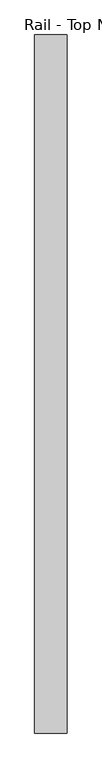
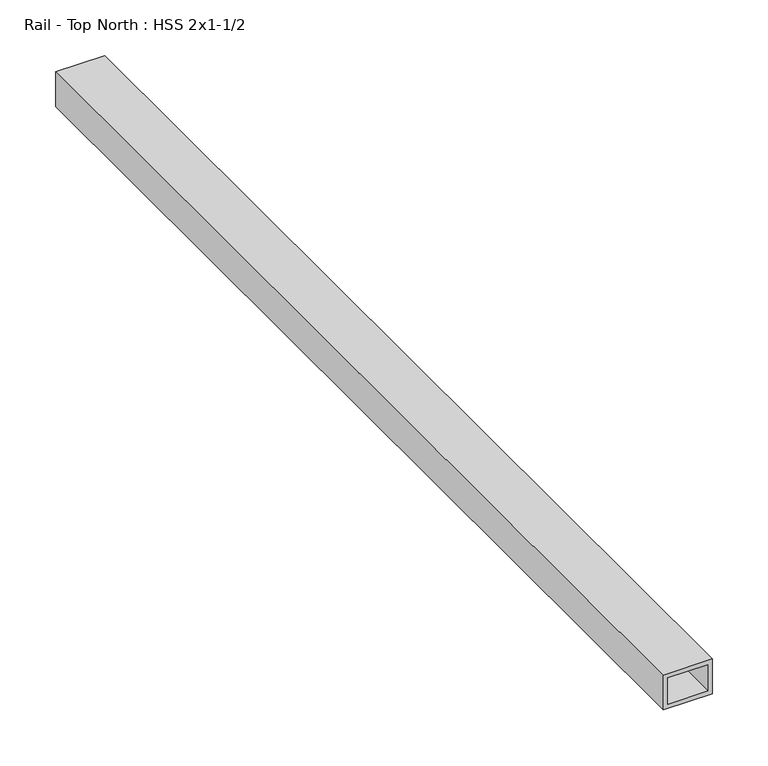
"""IFC4 building model written with IfcOpenShell, lengths in millimetres: proxy geometry, Rail - Top North : HSS 2x1-1/2."""

from ifc_helpers import new_model, si_unit, frame, origin, place, context, project, spatial, polyline, outline, extrude, source, transform, mapped, element, save


def rail_top_north_hss_2x1_1_2_493d1250(model_context):
    return source(origin(), model_context, "Body", "SweptSolid", [
        extrude(outline(polyline([(2400.3, 587416.6934739), (2438.4, 587416.6934739), (2438.4, 587365.8934739), (2400.3, 587365.8934739), (2400.3, 587416.6934739)]), holes=[polyline([(2433.6375, 587411.9309739), (2405.0625, 587411.9309739), (2405.0625, 587370.6559739), (2433.6375, 587370.6559739), (2433.6375, 587411.9309739)])]), frame((0.0, -532877.4663841, 0.0), z_axis=(0.0, 1.0, 0.0), x_axis=(0.0, 0.0, 1.0)), (0.0, 0.0, 1.0), 1092.2),
    ])


if __name__ == "__main__":
    model = new_model("IFC4")
    model_context = context("Model", 3, world=origin())
    ifc_project = project(units=[si_unit("LENGTHUNIT", "METRE", prefix="MILLI")], contexts=[model_context])
    site = spatial("IfcSite", under=ifc_project)
    building = spatial("IfcBuilding", under=site)
    placement = place(None, origin())
    rail_top_north_hss_2x1_1_2_shape = rail_top_north_hss_2x1_1_2_493d1250(model_context)
    element("IfcBuildingElementProxy", 1, Name="Rail - Top North : HSS 2x1-1/2", ObjectType="Rail - Top North : HSS 2x1-1/2", at=placement, inside=building, context=model_context, shape_type="MappedRepresentation", body=[
        mapped(rail_top_north_hss_2x1_1_2_shape, transform((0.0, 0.0, 0.0), x_axis=(1.0, 0.0, 0.0), y_axis=(0.0, 1.0, 0.0), z_axis=(0.0, 0.0, 1.0))),
    ])
    save(model, "model.ifc")

# Revit data of these elements
# Element 1 (IfcBuildingElementProxy, "Rail - Top North : HSS 2x1-1/2")
#   Materials on its faces: "1-1/2\"X2\" GALV. STL HSS TUBING"
# Materials
#   "1-1/2\"X2\" GALV. STL HSS TUBING": class "Generic", colour RGB 211 211 207, transparency 0, Cost = 0
